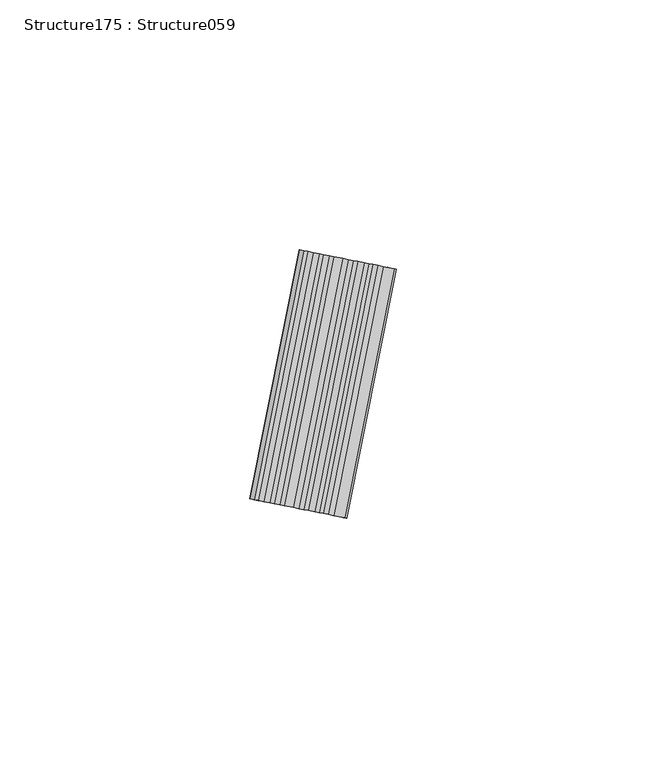
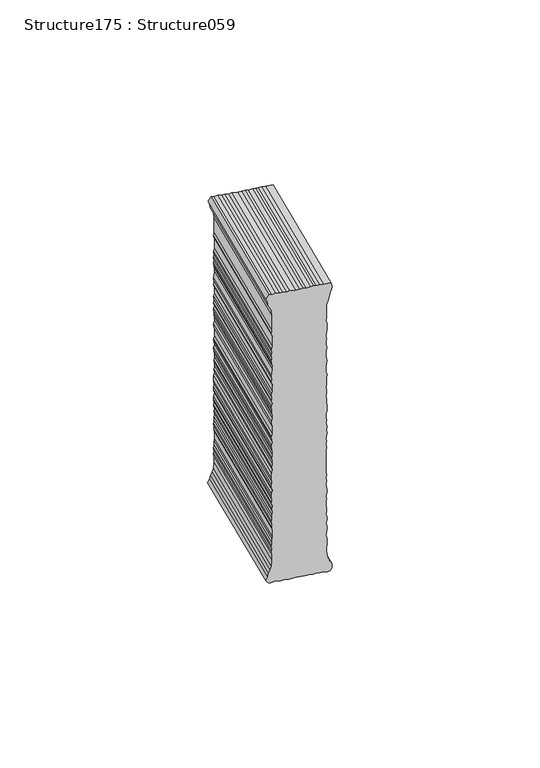
"""IFC4 building model written with IfcOpenShell, lengths in millimetres: proxy geometry, Structure175 : Structure059."""

from ifc_helpers import new_model, si_unit, frame, origin, place, context, project, spatial, polyline, outline, extrude, source, transform, mapped, element, save


def structure175_structure059_3b0decf3(model_context):
    return source(origin(), model_context, "Body", "SweptSolid", [
        extrude(outline(polyline([(1.8231554, 0.0), (3.146451, 0.2948314), (4.223301, 0.7409331), (5.4047307, 0.9167105), (6.4772964, 1.3627598), (7.4528114, 0.3820762), (7.3884057, -0.5247488), (7.0434645, -1.6749028), (7.2501163, -2.4718494), (7.1673846, -3.6367026), (6.9649918, -4.6632138), (7.0294228, -5.5791892), (6.8268536, -6.6081849), (6.629201, -7.5076866), (6.6888666, -8.5510265), (6.5229999, -10.8864115), (6.316449, -11.9112006), (6.523126, -12.7077923), (6.1783108, -13.8561717), (6.2561259, -14.6439679), (6.1641178, -15.9394323), (6.2193731, -16.9845991), (6.0352812, -17.7534372), (5.0780922, -18.3378809), (3.7953527, -18.1169333), (2.7962655, -17.5233917), (1.913164, -17.0697145), (1.0339666, -16.6163145), (-1.0179911, -16.2116048), (-2.0536528, -16.1380487), (-3.1025726, -16.1908973), (-5.1724761, -16.0438859), (-6.3290923, -15.7045498), (-7.5013464, -15.7511357), (-8.4171706, -15.8134371), (-9.3239956, -15.7490314), (-10.601995, -15.4010743), (-11.6561864, -15.5833915), (-12.6957522, -15.5095581), (-13.5787236, -15.1896572), (-14.500758, -15.2540145), (-15.6638365, -15.1714088), (-16.6906774, -14.968636), (-17.7302432, -14.8948027), (-18.7736607, -14.9505389), (-19.9293383, -14.7386157), (-20.9874337, -14.9206557), (-21.8942587, -14.85625), (-22.7920846, -14.6651372), (-23.8171509, -14.4624905), (-24.862343, -14.5181007), (-26.0258289, -14.3056229), (-26.9379254, -14.370686), (-28.097507, -14.1584856), (-35.4862676, -13.6337115), (-36.2730768, -13.7076729), (-37.56185, -13.4862968), (-38.6049127, -13.5420583), (-39.375855, -13.3574603), (-40.5481091, -13.4040461), (-41.4639333, -13.4663475), (-42.4948548, -13.2657818), (-43.6669324, -13.3098832), (-44.8136108, -12.971253), (-45.7335156, -13.0357615), (-46.8874186, -12.8239643), (-47.9269843, -12.750131), (-48.9811756, -12.9324482), (-50.9279214, -12.794184), (-51.822198, -12.6033233), (-53.1180172, -12.5112899), (-54.0160216, -12.3176676), (-55.1939545, -12.36385), (-56.2281963, -12.2903948), (-57.1258459, -12.0967976), (-58.0414915, -12.1616086), (-60.3797159, -11.9955402), (-61.418343, -12.0491198), (-62.4404439, -11.7193374), (-64.2597726, -11.5901227), (-65.4323817, -11.6366833), (-66.3425272, -11.6993881), (-67.4987884, -11.3600772), (-69.568692, -11.2130658), (-70.4940467, -11.4045335), (-71.7716912, -11.0566016), (-72.8073528, -10.9830455), (-73.5945168, -11.0569817), (-74.7487746, -10.8451594), (-75.7996455, -10.9003662), (-76.7154697, -10.9626676), (-78.918114, -10.8062286), (-79.8067643, -10.4859243), (-80.9846972, -10.5321068), (-85.2575999, -10.2286312), (-87.1143914, -10.616842), (-88.4338333, -10.9126605), (-89.3541939, -10.9785635), (-90.2847425, -11.3034293), (-91.3371067, -11.4901569), (-92.6113068, -11.0083459), (-92.4548678, -8.8057016), (-92.5012015, -7.6298983), (-92.2982775, -6.6009278), (-92.3722137, -5.8137637), (-92.3077828, -4.9065838), (-91.9594959, -3.6289645), (-92.1513185, -2.7035847), (-91.948571, -1.6770986), (-91.7387772, -0.5212698), (-91.8660681, 1.3127098), (-91.5453837, 2.2016897), (-91.7187795, 3.3865175), (-91.5250311, 4.2862964), (-91.5714908, 5.4603251), (-91.2323544, 6.6091078), (-91.4333526, 7.4052963), (-89.9470277, 8.0820021), (-89.2007223, 7.6359003), (-87.9140786, 7.4146755), (-85.9177564, 6.2316476), (-83.8509695, 5.9553711), (-78.9274953, 5.6056898), (-77.7492326, 5.6514922), (-76.8612147, 5.327309), (-73.4894581, 5.0878358), (-72.4346346, 5.274032), (-71.4102529, 5.0717906), (-70.4939226, 5.1361963), (-69.3343157, 4.9243507), (-68.4179854, 4.9887564), (-67.3911192, 4.7863385), (-66.4932409, 4.5909415), (-65.4536751, 4.5171081), (-63.3653195, 4.6298995), (-62.2057127, 4.4180539), (-61.0331289, 4.4642596), (-60.139432, 4.1396731), (-57.9421116, 3.9836122), (-57.1438965, 4.1880336), (-55.8572276, 3.9671637), (-54.8117057, 4.0223937), (-53.9197836, 3.6979333), (-52.8653149, 3.8841547), (-51.7113868, 3.6727125), (-50.8045618, 3.6083068), (-49.777492, 3.4037341), (-48.7379263, 3.3299008), (-47.5507169, 3.5066945), (-45.755164, 3.1180552), (-43.4233281, 2.9524405), (-42.3709891, 3.1388132), (-41.6000215, 2.9545701), (-40.5694025, 2.7497454), (-39.5170634, 2.936118), (-38.2342987, 2.7155254), (-37.2036797, 2.5107007), (-36.1676632, 2.4371194), (-35.122345, 2.4945043), (-34.0920809, 2.2897047), (-33.0578389, 2.2162495), (-32.0089715, 2.2733822), (-30.9822567, 2.0688348), (-29.927788, 2.2550562), (-28.1137831, 2.1262196), (-26.9559508, 1.9145001), (-26.0399754, 1.978931), (-24.8751223, 1.8961993), (-23.9828452, 1.5717136), (-22.8013146, 1.7489107), (-21.765298, 1.6753294), (-20.8615898, 1.4816586), (-19.8185523, 1.5370651), (-18.6682471, 1.1942534), (-17.7517654, 1.2607887), (-16.7250506, 1.0562412), (-15.6818619, 1.1137773), (-14.3860427, 1.021744), (-13.4697123, 1.0861496), (-12.4371674, 0.8833285), (-11.2740889, 0.8007228), (-10.5057571, 0.6145266), (-8.1735663, 0.4488867), (-7.3845017, 0.5244716), (-6.0886824, 0.4324382), (-5.0435154, 0.4876935), (-4.0127452, 0.2849983), (-3.2295105, 0.3588569), (-1.9428416, 0.137987), (0.0, 0.0), (1.8231554, 0.0)])), frame((-1717.0136786, 234809.2341358, 393.8064615), z_axis=(0.19466222296394123, 0.9808703374813293, 0.0), x_axis=(-0.06948958876060478, 0.0137908113887096, -0.9974873485789798)), (0.0, 0.0, 1.0), 50.8),
    ])


if __name__ == "__main__":
    model = new_model("IFC4")
    model_context = context("Model", 3, world=origin())
    ifc_project = project(units=[si_unit("LENGTHUNIT", "METRE", prefix="MILLI")], contexts=[model_context])
    site = spatial("IfcSite", under=ifc_project)
    building = spatial("IfcBuilding", under=site)
    placement = place(None, origin())
    structure175_structure059_shape = structure175_structure059_3b0decf3(model_context)
    element("IfcBuildingElementProxy", 1, Name="Structure175 : Structure059", ObjectType="Structure175 : Structure059", at=placement, inside=building, context=model_context, shape_type="MappedRepresentation", body=[
        mapped(structure175_structure059_shape, transform((0.0, 0.0, 0.0), x_axis=(1.0, 0.0, 0.0), y_axis=(0.0, 1.0, 0.0), z_axis=(0.0, 0.0, 1.0))),
    ])
    save(model, "model.ifc")

# Revit data of these elements
# Type "Structure175 : Structure059"
#   NameOverride = "Structure059"
# Element 1 (IfcBuildingElementProxy, "Structure175 : Structure059")
#   Materials on its faces: "BRUSHED ALUMINUM LETTERING"
# Materials
#   "BRUSHED ALUMINUM LETTERING": class "Unassigned", colour RGB 169 181 186, transparency 0, Cost = 0
